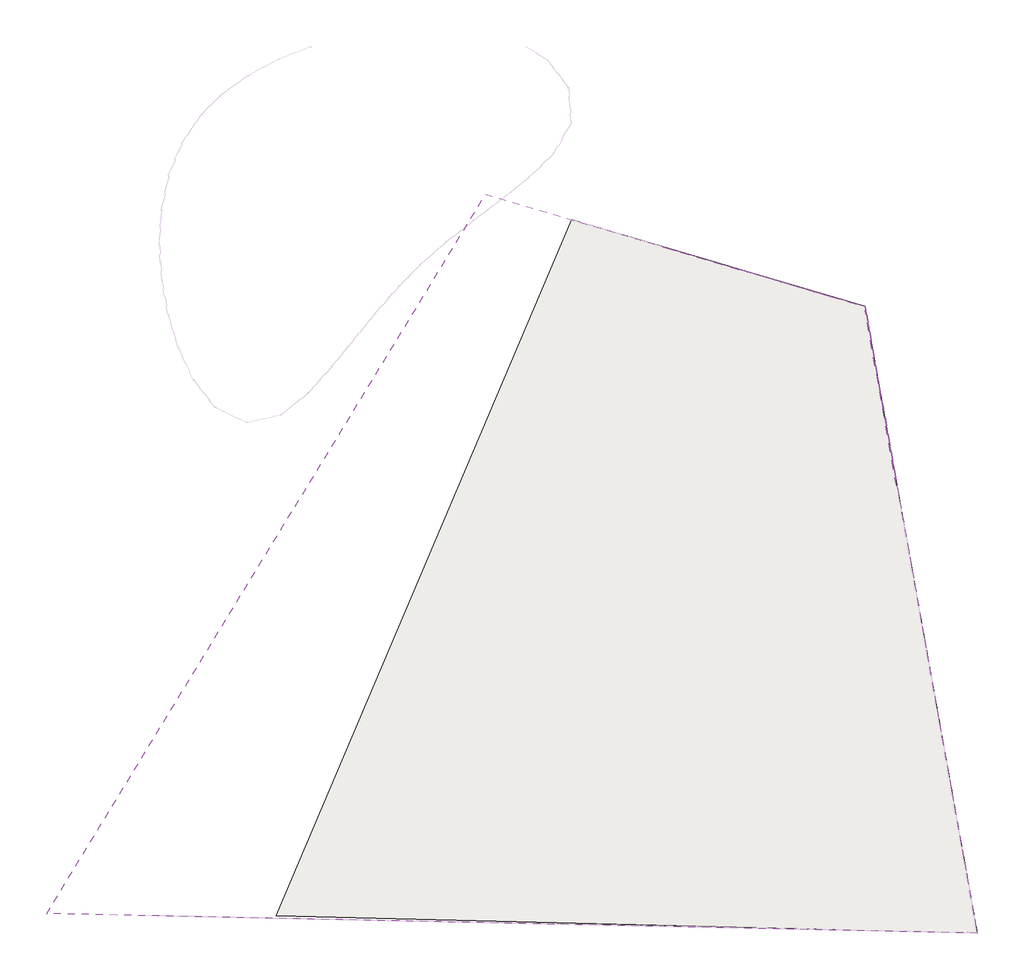
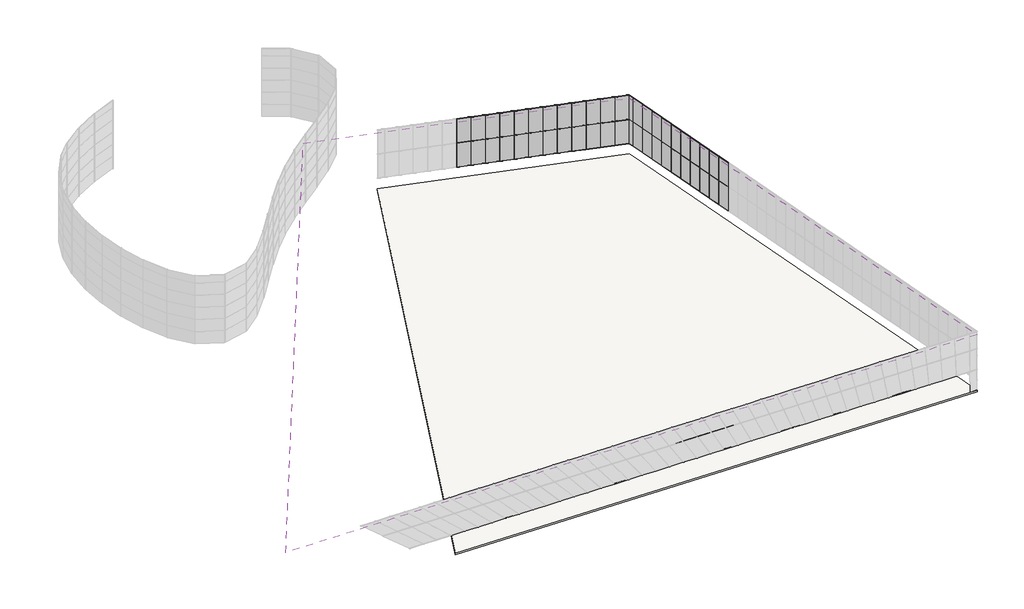
# One storey, part 8 of 8: 69 members, 46 plates, 1 roof, 1 slab.
# Revit data of these elements (continued)
# Type "Montante circular : 25 mm Raio"
#   built-in parameter 1007350 = 0.082021 (stored number, unit not read)
# Type "Painel do sistema : Envidraçado"
#   Construction Type Id = "GSP4R"
#   Analytic Construction = "Vidraça única Pilkington 1/8 pol"
#   Visual Light Transmittance = 0.9
#   Solar Heat Gain Coefficient = 0.86
#   Heat Transfer Coefficient (U) = 6.7069 W/(m²·K)
# Type "Genérico - 400 mm"
#   Layers, outside or top first: 400 mm no material (function 1)
# Type "Genérico 150 mm"
#   Function = 0
#   Layers, outside or top first: 150 mm no material (function 1)
# Elements 1, 2, 3, 4, 5, 6, 7, 8, 9, 10, 11, 12, 13, 14, 15, 16, 17, 18, 19, 20, 21, 22, 23, 24, 25, 26, 27, 28, 29, 30, 31, 32, 33, 34, 35, 36, 37, 38, 39, 40, 41, 42, 43, 44, 45, 46, 47, 48, 49, 50, 51, 52, 53, 54, 55, 56, 57, 58, 59, 60, 61, 62, 63, 64, 65, 66, 67, 68, 69 (IfcMember, "Montante circular : 25 mm Raio")
#   Phase Created = Construção nova
#   Materials on its faces: "Alumín."
# Elements 70, 71, 72, 73, 74, 75, 76, 77, 78, 79, 80, 81, 82, 83, 84, 85, 86, 87, 88, 89, 90, 91, 92, 93, 94, 95, 96, 97, 98, 99, 100, 101, 102, 103, 104, 105, 106, 107, 108, 109, 110, 111, 112, 113, 114, 115 (IfcPlate, "Painel do sistema : Envidraçado")
#   Phase Created = Construção nova
#   Materials on its faces: "Vidro"
# Element 116 (IfcRoof, "Genérico - 400 mm")
#   built-in parameter 1001710 = 33615
#   Phase Created = Construção nova
#   Materials on its faces: "Material pré-definido de cobertura"
# Element 117 (IfcSlab, "Genérico 150 mm")
#   built-in parameter 1001955 = -0.287112 (stored number, unit not read)
#   Height Offset From Level = 0 mm
#   Phase Created = Construção nova
#   Materials on its faces: "Material pré-definido de piso"
# Materials
#   "Alumín.": class "Metal", colour RGB 247 247 247, transparency 0, Description = "Alumín. 6061", Cost = 0
#   "Vidro": class "Vidro", colour RGB 0 128 192, transparency 0.9, Description = "Vidro de sílica", Cost = 0
#   "Material pré-definido de cobertura": class "Diversos", colour RGB 0 127 0, transparency 0, Cost = 0
#   "Material pré-definido de piso": class "Diversos", colour RGB 127 127 127, transparency 0, Cost = 0
